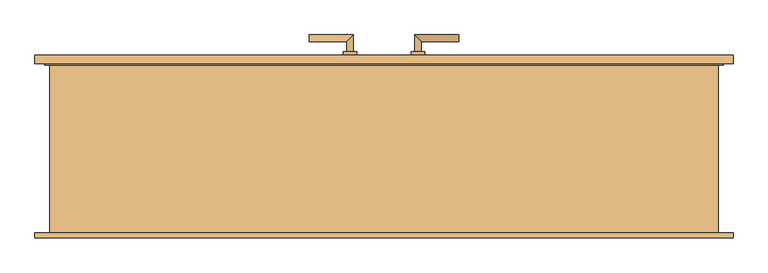
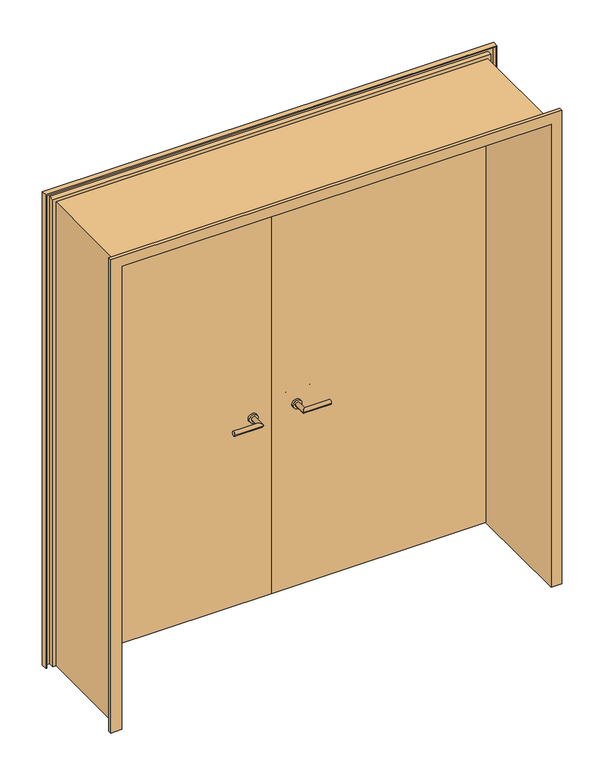
"""IFC4 building model written with IfcOpenShell, lengths in millimetres: door geometry, Drehflügel 2-flg - Variabel : Drehflügel 2-flg - Variabel."""

from ifc_helpers import new_model, si_unit, point, frame, frame_2d, origin, origin_with_axes, place, context, project, spatial, polyline, circle_curve, ellipse_curve, trimmed, segment, composite_curve, outline, extrude, faceted_brep, source, transform, mapped, element, save
from ifc_brep_helpers import plane_surface, cylinder_surface, advanced_brep


def door_da8c1179(model_context):
    return source(origin(), model_context, "Body", "SolidModel", [
        advanced_brep(
        [(-90.0, 239.4346141, 900.0), (-110.0, 239.4346141, 900.0), (-110.0, 189.4346141, 900.0), (-90.0, 169.4346141, 900.0), (-220.0, 169.4346141, 900.0), (-220.0, 189.4346141, 900.0)],
        [
            (0, 1, circle_curve(frame((-100.0, 239.4346141, 900.0), z_axis=(0.0, 1.0, 0.0), x_axis=(-1.0, 0.0, 0.0)), 10.0)),
            (1, 0, circle_curve(frame((-100.0, 239.4346141, 900.0), z_axis=(0.0, 1.0, 0.0), x_axis=(-1.0, 0.0, 0.0)), 10.0)),
            (1, 2),
            (2, 3, ellipse_curve(frame((-100.0, 179.4346141, 900.0), z_axis=(0.7071067811865385, 0.7071067811865565, 0.0), x_axis=(-0.7071067811865563, 0.7071067811865386, 0.0)), 14.1421356, 10.0)),
            (3, 0),
            (3, 2, ellipse_curve(frame((-100.0, 179.4346141, 900.0), z_axis=(0.7071067811865385, 0.7071067811865565, 0.0), x_axis=(-0.7071067811865563, 0.7071067811865386, 0.0)), 14.1421356, 10.0)),
            (4, 5, circle_curve(frame((-220.0, 179.4346141, 900.0), z_axis=(-1.0, 0.0, 0.0), x_axis=(0.0, 1.0, 0.0)), 10.0)),
            (5, 4, circle_curve(frame((-220.0, 179.4346141, 900.0), z_axis=(-1.0, 0.0, 0.0), x_axis=(0.0, 1.0, 0.0)), 10.0)),
            (2, 5),
            (4, 3),
        ],
        [
            plane_surface(frame((-100.0, 239.4346141, -387.7526403), z_axis=(0.0, 1.0, 0.0), x_axis=(0.0, 0.0, 1.0))),
            cylinder_surface(frame((-100.0, 239.4346141, 900.0), z_axis=(0.0, 1.0, 0.0), x_axis=(-1.0, 0.0, 0.0)), 10.0),
            plane_surface(frame((-220.0, 179.4346141, -387.7526403), z_axis=(-1.0, 0.0, 0.0), x_axis=(0.0, 0.0, 1.0))),
            cylinder_surface(frame((-100.0, 179.4346141, 900.0), z_axis=(1.0, 0.0, 0.0), x_axis=(0.0, 1.0, 0.0)), 10.0),
        ],
        [
            (0, [[1, 2]]),
            (1, [[3, 4, 5, -2]]),
            (1, [[-5, 6, -3, -1]]),
            (2, [[7, 8]]),
            (3, [[9, -7, 10, -4]]),
            (3, [[-10, -8, -9, -6]]),
        ],
    ),
        advanced_brep(
        [(-110.0, 299.4346141, 900.0), (-90.0, 299.4346141, 900.0), (-90.0, 349.4346141, 900.0), (-110.0, 329.4346141, 900.0), (-220.0, 329.4346141, 900.0), (-220.0, 349.4346141, 900.0)],
        [
            (0, 1, circle_curve(frame((-100.0, 299.4346141, 900.0), z_axis=(0.0, -1.0, 0.0), x_axis=(1.0, 0.0, 0.0)), 10.0)),
            (1, 0, circle_curve(frame((-100.0, 299.4346141, 900.0), z_axis=(0.0, -1.0, 0.0), x_axis=(1.0, 0.0, 0.0)), 10.0)),
            (1, 2),
            (2, 3, ellipse_curve(frame((-100.0, 339.4346141, 900.0), z_axis=(0.7071067811865475, -0.7071067811865475, 0.0), x_axis=(-0.7071067811865474, -0.7071067811865476, 0.0)), 14.1421356, 10.0)),
            (3, 0),
            (3, 2, ellipse_curve(frame((-100.0, 339.4346141, 900.0), z_axis=(0.7071067811865475, -0.7071067811865475, 0.0), x_axis=(-0.7071067811865474, -0.7071067811865476, 0.0)), 14.1421356, 10.0)),
            (4, 5, circle_curve(frame((-220.0, 339.4346141, 900.0), z_axis=(-1.0, 0.0, 0.0), x_axis=(0.0, 1.0, 0.0)), 10.0)),
            (5, 4, circle_curve(frame((-220.0, 339.4346141, 900.0), z_axis=(-1.0, 0.0, 0.0), x_axis=(0.0, 1.0, 0.0)), 10.0)),
            (2, 5),
            (4, 3),
        ],
        [
            plane_surface(frame((-100.0, 299.4346141, -387.7526403), z_axis=(0.0, -1.0, 0.0), x_axis=(0.0, 0.0, 1.0))),
            cylinder_surface(frame((-100.0, 299.4346141, 900.0), z_axis=(0.0, -1.0, 0.0), x_axis=(1.0, 0.0, 0.0)), 10.0),
            plane_surface(frame((-220.0, 339.4346141, -387.7526403), z_axis=(-1.0, 0.0, 0.0), x_axis=(0.0, 0.0, 1.0))),
            cylinder_surface(frame((-100.0, 339.4346141, 900.0), z_axis=(1.0, 0.0, 0.0), x_axis=(0.0, 1.0, 0.0)), 10.0),
        ],
        [
            (0, [[1, 2]]),
            (1, [[3, 4, 5, -2]]),
            (1, [[-5, 6, -3, -1]]),
            (2, [[7, 8]]),
            (3, [[9, -7, 10, -4]]),
            (3, [[-10, -8, -9, -6]]),
        ],
    ),
        extrude(outline(composite_curve([segment(trimmed(circle_curve(frame_2d((900.0, -100.0)), 20.0), [point((900.0, -80.0))], [point((900.0, -120.0))], False, "CARTESIAN"), True, "CONTINUOUS"), segment(trimmed(circle_curve(frame_2d((900.0, -100.0)), 20.0), [point((900.0, -120.0))], [point((900.0, -80.0))], False, "CARTESIAN"), True, "CONTINUOUS")], self_intersect=False)), frame((0.0, 229.4346141, 0.0), z_axis=(0.0, 1.0, 0.0), x_axis=(0.0, 0.0, 1.0)), (0.0, 0.0, 1.0), 10.0),
        extrude(outline(composite_curve([segment(trimmed(circle_curve(frame_2d((900.0, -100.0)), 20.0), [point((900.0, -80.0))], [point((900.0, -120.0))], False, "CARTESIAN"), True, "CONTINUOUS"), segment(trimmed(circle_curve(frame_2d((900.0, -100.0)), 20.0), [point((900.0, -120.0))], [point((900.0, -80.0))], False, "CARTESIAN"), True, "CONTINUOUS")], self_intersect=False)), frame((0.0, 289.4346141, 0.0), z_axis=(0.0, 1.0, 0.0), x_axis=(0.0, 0.0, 1.0)), (0.0, 0.0, 1.0), 10.0),
        advanced_brep(
        [(90.0, 239.4346141, 900.0), (110.0, 239.4346141, 900.0), (90.0, 169.4346141, 900.0), (110.0, 189.4346141, 900.0), (220.0, 169.4346141, 900.0), (220.0, 189.4346141, 900.0)],
        [
            (0, 1, circle_curve(frame((100.0, 239.4346141, 900.0), z_axis=(0.0, 1.0, 0.0), x_axis=(1.0, 0.0, 0.0)), 10.0)),
            (1, 0, circle_curve(frame((100.0, 239.4346141, 900.0), z_axis=(0.0, 1.0, 0.0), x_axis=(1.0, 0.0, 0.0)), 10.0)),
            (0, 2),
            (2, 3, ellipse_curve(frame((100.0, 179.4346141, 900.0), z_axis=(-0.7071067811865385, 0.7071067811865565, 0.0), x_axis=(0.7071067811865563, 0.7071067811865386, 0.0)), 14.1421356, 10.0)),
            (3, 1),
            (3, 2, ellipse_curve(frame((100.0, 179.4346141, 900.0), z_axis=(-0.7071067811865385, 0.7071067811865565, 0.0), x_axis=(0.7071067811865563, 0.7071067811865386, 0.0)), 14.1421356, 10.0)),
            (4, 5, circle_curve(frame((220.0, 179.4346141, 900.0), z_axis=(1.0, 0.0, 0.0), x_axis=(0.0, 1.0, 0.0)), 10.0)),
            (5, 4, circle_curve(frame((220.0, 179.4346141, 900.0), z_axis=(1.0, 0.0, 0.0), x_axis=(0.0, 1.0, 0.0)), 10.0)),
            (2, 4),
            (5, 3),
        ],
        [
            plane_surface(frame((100.0, 239.4346141, -387.7526403), z_axis=(0.0, 1.0, 0.0), x_axis=(0.0, 0.0, 1.0))),
            cylinder_surface(frame((100.0, 239.4346141, 900.0), z_axis=(0.0, 1.0, 0.0), x_axis=(1.0, 0.0, 0.0)), 10.0),
            plane_surface(frame((220.0, 179.4346141, -387.7526403), z_axis=(1.0, 0.0, 0.0), x_axis=(0.0, 0.0, 1.0))),
            cylinder_surface(frame((100.0, 179.4346141, 900.0), z_axis=(-1.0, 0.0, 0.0), x_axis=(0.0, 1.0, 0.0)), 10.0),
        ],
        [
            (0, [[1, 2]]),
            (1, [[-1, 3, 4, 5]]),
            (1, [[-2, -5, 6, -3]]),
            (2, [[7, 8]]),
            (3, [[-4, 9, -8, 10]]),
            (3, [[-6, -10, -7, -9]]),
        ],
    ),
        advanced_brep(
        [(110.0, 299.4346141, 900.0), (90.0, 299.4346141, 900.0), (110.0, 329.4346141, 900.0), (90.0, 349.4346141, 900.0), (220.0, 329.4346141, 900.0), (220.0, 349.4346141, 900.0)],
        [
            (0, 1, circle_curve(frame((100.0, 299.4346141, 900.0), z_axis=(0.0, -1.0, 0.0), x_axis=(-1.0, 0.0, 0.0)), 10.0)),
            (1, 0, circle_curve(frame((100.0, 299.4346141, 900.0), z_axis=(0.0, -1.0, 0.0), x_axis=(-1.0, 0.0, 0.0)), 10.0)),
            (0, 2),
            (2, 3, ellipse_curve(frame((100.0, 339.4346141, 900.0), z_axis=(-0.7071067811865475, -0.7071067811865475, 0.0), x_axis=(0.7071067811865474, -0.7071067811865476, 0.0)), 14.1421356, 10.0)),
            (3, 1),
            (3, 2, ellipse_curve(frame((100.0, 339.4346141, 900.0), z_axis=(-0.7071067811865475, -0.7071067811865475, 0.0), x_axis=(0.7071067811865474, -0.7071067811865476, 0.0)), 14.1421356, 10.0)),
            (4, 5, circle_curve(frame((220.0, 339.4346141, 900.0), z_axis=(1.0, 0.0, 0.0), x_axis=(0.0, 1.0, 0.0)), 10.0)),
            (5, 4, circle_curve(frame((220.0, 339.4346141, 900.0), z_axis=(1.0, 0.0, 0.0), x_axis=(0.0, 1.0, 0.0)), 10.0)),
            (2, 4),
            (5, 3),
        ],
        [
            plane_surface(frame((100.0, 299.4346141, -387.7526403), z_axis=(0.0, -1.0, 0.0), x_axis=(0.0, 0.0, 1.0))),
            cylinder_surface(frame((100.0, 299.4346141, 900.0), z_axis=(0.0, -1.0, 0.0), x_axis=(-1.0, 0.0, 0.0)), 10.0),
            plane_surface(frame((220.0, 339.4346141, -387.7526403), z_axis=(1.0, 0.0, 0.0), x_axis=(0.0, 0.0, 1.0))),
            cylinder_surface(frame((100.0, 339.4346141, 900.0), z_axis=(-1.0, 0.0, 0.0), x_axis=(0.0, 1.0, 0.0)), 10.0),
        ],
        [
            (0, [[1, 2]]),
            (1, [[-1, 3, 4, 5]]),
            (1, [[-2, -5, 6, -3]]),
            (2, [[7, 8]]),
            (3, [[-4, 9, -8, 10]]),
            (3, [[-6, -10, -7, -9]]),
        ],
    ),
        extrude(outline(composite_curve([segment(trimmed(circle_curve(frame_2d((900.0, 100.0)), 20.0), [point((900.0, 80.0))], [point((900.0, 120.0))], False, "CARTESIAN"), True, "CONTINUOUS"), segment(trimmed(circle_curve(frame_2d((900.0, 100.0)), 20.0), [point((900.0, 120.0))], [point((900.0, 80.0))], False, "CARTESIAN"), True, "CONTINUOUS")], self_intersect=False)), frame((0.0, 229.4346141, 0.0), z_axis=(0.0, 1.0, 0.0), x_axis=(0.0, 0.0, 1.0)), (0.0, 0.0, 1.0), 10.0),
        extrude(outline(composite_curve([segment(trimmed(circle_curve(frame_2d((900.0, 100.0)), 20.0), [point((900.0, 80.0))], [point((900.0, 120.0))], False, "CARTESIAN"), True, "CONTINUOUS"), segment(trimmed(circle_curve(frame_2d((900.0, 100.0)), 20.0), [point((900.0, 120.0))], [point((900.0, 80.0))], False, "CARTESIAN"), True, "CONTINUOUS")], self_intersect=False)), frame((0.0, 289.4346141, 0.0), z_axis=(0.0, 1.0, 0.0), x_axis=(0.0, 0.0, 1.0)), (0.0, 0.0, 1.0), 10.0),
        extrude(outline(polyline([(0.0, 264.4346141), (-995.0, 264.4346141), (-995.0, 289.4346141), (0.0, 289.4346141), (0.0, 264.4346141)])), origin_with_axes(), (0.0, 0.0, 1.0), 2250.0),
        extrude(outline(polyline([(995.0, 264.4346141), (0.0, 264.4346141), (0.0, 289.4346141), (995.0, 289.4346141), (995.0, 264.4346141)])), origin_with_axes(), (0.0, 0.0, 1.0), 2250.0),
        faceted_brep([(1029.5, -250.5653859, 0.0), (980.0, -250.5653859, 0.0), (980.0, 264.4346141, 0.0), (995.0, 264.4346141, 0.0), (995.0, 289.4346141, 0.0), (1029.5, 289.4346141, 0.0), (1029.5, 264.4346141, 0.0), (1024.5, 264.4346141, 0.0), (1024.5, 284.4346141, 0.0), (1000.0, 284.4346141, 0.0), (1000.0, 259.4346141, 0.0), (985.0, 259.4346141, 0.0), (985.0, -245.5653859, 0.0), (1024.5, -245.5653859, 0.0), (1024.5, -235.5653859, 0.0), (1029.5, -235.5653859, 0.0), (1029.5, -250.5653859, 2284.5), (-1029.5, -250.5653859, 2284.5), (-1029.5, -250.5653859, 0.0), (-980.0, -250.5653859, 0.0), (-980.0, -250.5653859, 2235.0), (980.0, -250.5653859, 2235.0), (980.0, 264.4346141, 2235.0), (-980.0, 264.4346141, 2235.0), (-980.0, 264.4346141, 0.0), (-995.0, 264.4346141, 0.0), (-995.0, 264.4346141, 2250.0), (995.0, 264.4346141, 2250.0), (995.0, 289.4346141, 2250.0), (-995.0, 289.4346141, 2250.0), (-995.0, 289.4346141, 0.0), (-1029.5, 289.4346141, 0.0), (-1029.5, 289.4346141, 2284.5), (1029.5, 289.4346141, 2284.5), (1029.5, 264.4346141, 2284.5), (-1029.5, 264.4346141, 2284.5), (-1029.5, 264.4346141, 0.0), (-1024.5, 264.4346141, 0.0), (-1024.5, 264.4346141, 2279.5), (1024.5, 264.4346141, 2279.5), (1024.5, 284.4346141, 2279.5), (-1024.5, 284.4346141, 2279.5), (-1024.5, 284.4346141, 0.0), (-1000.0, 284.4346141, 0.0), (-1000.0, 284.4346141, 2255.0), (1000.0, 284.4346141, 2255.0), (1000.0, 259.4346141, 2255.0), (-1000.0, 259.4346141, 2255.0), (-1000.0, 259.4346141, 0.0), (-985.0, 259.4346141, 0.0), (-985.0, 259.4346141, 2240.0), (985.0, 259.4346141, 2240.0), (985.0, -245.5653859, 2240.0), (-985.0, -245.5653859, 2240.0), (-985.0, -245.5653859, 0.0), (-1024.5, -245.5653859, 0.0), (-1024.5, -245.5653859, 2279.5), (1024.5, -245.5653859, 2279.5), (1024.5, -235.5653859, 2279.5), (-1024.5, -235.5653859, 2279.5), (-1024.5, -235.5653859, 0.0), (-1029.5, -235.5653859, 0.0), (-1029.5, -235.5653859, 2284.5), (1029.5, -235.5653859, 2284.5)], [[[0, 1, 2, 3, 4, 5, 6, 7, 8, 9, 10, 11, 12, 13, 14, 15]], [[1, 0, 16, 17, 18, 19, 20, 21]], [[2, 1, 21, 22]], [[3, 2, 22, 23, 24, 25, 26, 27]], [[4, 3, 27, 28]], [[5, 4, 28, 29, 30, 31, 32, 33]], [[6, 5, 33, 34]], [[7, 6, 34, 35, 36, 37, 38, 39]], [[8, 7, 39, 40]], [[9, 8, 40, 41, 42, 43, 44, 45]], [[10, 9, 45, 46]], [[11, 10, 46, 47, 48, 49, 50, 51]], [[12, 11, 51, 52]], [[13, 12, 52, 53, 54, 55, 56, 57]], [[14, 13, 57, 58]], [[15, 14, 58, 59, 60, 61, 62, 63]], [[0, 15, 63, 16]], [[17, 62, 61, 18]], [[18, 61, 60, 55, 54, 49, 48, 43, 42, 37, 36, 31, 30, 25, 24, 19]], [[23, 20, 19, 24]], [[29, 26, 25, 30]], [[35, 32, 31, 36]], [[41, 38, 37, 42]], [[47, 44, 43, 48]], [[53, 50, 49, 54]], [[59, 56, 55, 60]], [[22, 21, 20, 23]], [[28, 27, 26, 29]], [[34, 33, 32, 35]], [[40, 39, 38, 41]], [[46, 45, 44, 47]], [[52, 51, 50, 53]], [[58, 57, 56, 59]], [[16, 63, 62, 17]]]),
    ])


if __name__ == "__main__":
    model = new_model("IFC4")
    model_context = context("Model", 3, world=origin())
    ifc_project = project(units=[si_unit("LENGTHUNIT", "METRE", prefix="MILLI")], contexts=[model_context])
    site = spatial("IfcSite", under=ifc_project)
    building = spatial("IfcBuilding", under=site)
    placement = place(None, origin())
    door_shape = door_da8c1179(model_context)
    element("IfcDoor", 1, ObjectType="Drehflügel 2-flg - Variabel : Drehflügel 2-flg - Variabel", at=placement, inside=building, context=model_context, shape_type="MappedRepresentation", body=[
        mapped(door_shape, transform((0.0, 0.0, 0.0), x_axis=(1.0, 0.0, 0.0), y_axis=(0.0, 1.0, 0.0), z_axis=(0.0, 0.0, 1.0))),
    ])
    save(model, "model.ifc")

# Revit data of these elements
# Type "Drehflügel 2-flg - Variabel : Drehflügel 2-flg - Variabel"
#   Construction Type Id = "MDOOR"
#   Type Mark = "18"
#   Operation = "DoubleDoorSingleSwing"
#   Keynote = "16.03"
#   Analytic Construction = "Metall"
#   Thermal Resistance (R) = 0.270117 (m²·K)/W
#   Heat Transfer Coefficient (U) = 3.7021 W/(m²·K)
#   Rough Width [instance default] = 2.010 m
#   Rough Height [instance default] = 2.360 m
#   Höhe Türgriff = 0.900 m
#   Height [instance default] = 2.260 m
#   Fußbodenaufbau [instance default] = 0.100 m
#   Width [instance default] = 2.010 m
#   Sichtbarkeit Sturzlinien [instance default] = yes
#   Türgriff auswählen [instance default] = element 222671
#   Türgriff [instance default] = none
#   Türflügel [instance default] = none
#   Rahmen/Pfosten [instance default] = Metall - Lackiert - Grau
#   Visual Light Transmittance = 0
#   Solar Heat Gain Coefficient = 0
#   Function = (empty or 0)
#   Wall Closure = (empty or 0)
# Element 1 (IfcDoor, "Drehflügel 2-flg - Variabel : Drehflügel 2-flg - Variabel")
#   Rough Height = 2.260 m
#   Fußbodenaufbau = 0.000 m
#   Materials on its faces: "Metall - Chrom", "Metall - Lackiert - Grau", "Holz - Birke"
# Materials
#   "Metall - Lackiert - Grau": class "Farbe 1", colour RGB 98 98 98, transparency 0, Cost = 0
#   "Metall - Chrom": class "Metall", colour RGB 247 247 247, transparency 0, Cost = 0
#   "Holz - Birke": class "Holz", colour RGB 213 164 103, transparency 0, Cost = 0
